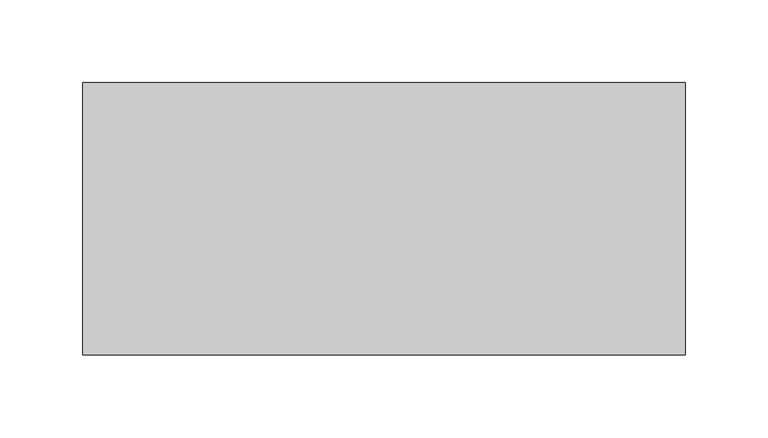
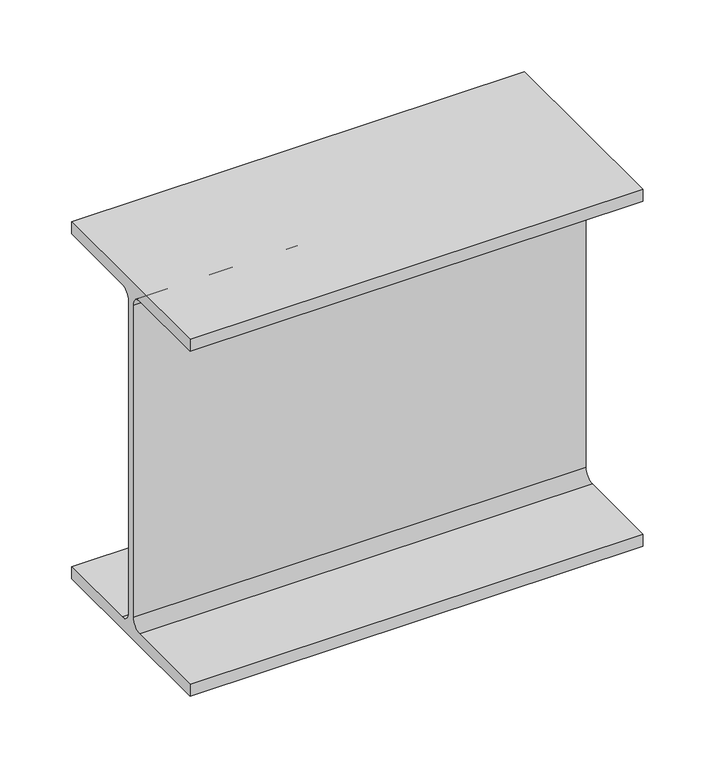
"""IFC4 building model written with IfcOpenShell, lengths in millimetres: beam geometry, Steel Beam_H-KSD3502 : H_SB_ASB_H-300x150x6.5x9."""

from ifc_helpers import new_model, si_unit, point, frame, frame_2d, origin, place, context, project, spatial, polyline, circle_curve, trimmed, segment, composite_curve, outline, extrude, source, transform, mapped, element, save


def beam_067efcca(model_context):
    return source(origin(), model_context, "Body", "SweptSolid", [
        extrude(outline(composite_curve([segment(polyline([(82.5, -141.5), (82.5, -151.7), (-82.5, -151.7), (-82.5, -141.5), (-11.9, -141.5)]), True, "CONTINUOUS"), segment(trimmed(circle_curve(frame_2d((-11.9, -132.6)), 8.9), [point((-11.9, -141.5))], [point((-3.0, -132.6))], True, "CARTESIAN"), True, "CONTINUOUS"), segment(polyline([(-3.0, -132.6), (-3.0, 132.6)]), True, "CONTINUOUS"), segment(trimmed(circle_curve(frame_2d((-11.9, 132.6)), 8.9), [point((-3.0, 132.6))], [point((-11.9, 141.5))], True, "CARTESIAN"), True, "CONTINUOUS"), segment(polyline([(-11.9, 141.5), (-82.5, 141.5), (-82.5, 151.7), (82.5, 151.7), (82.5, 141.5), (11.9, 141.5)]), True, "CONTINUOUS"), segment(trimmed(circle_curve(frame_2d((11.9, 132.6)), 8.9), [point((11.9, 141.5))], [point((3.0, 132.6))], True, "CARTESIAN"), True, "CONTINUOUS"), segment(polyline([(3.0, 132.6), (3.0, -132.6)]), True, "CONTINUOUS"), segment(trimmed(circle_curve(frame_2d((11.9, -132.6)), 8.9), [point((3.0, -132.6))], [point((11.9, -141.5))], True, "CARTESIAN"), True, "CONTINUOUS"), segment(polyline([(11.9, -141.5), (82.5, -141.5)]), True, "CONTINUOUS")], self_intersect=False)), frame((-282.3, 0.0, 0.0), z_axis=(1.0, 0.0, 0.0), x_axis=(0.0, 1.0, 0.0)), (0.0, 0.0, 1.0), 364.6),
    ])


if __name__ == "__main__":
    model = new_model("IFC4")
    model_context = context("Model", 3, world=origin())
    ifc_project = project(units=[si_unit("LENGTHUNIT", "METRE", prefix="MILLI")], contexts=[model_context])
    site = spatial("IfcSite", under=ifc_project)
    building = spatial("IfcBuilding", under=site)
    placement = place(None, origin())
    beam_shape = beam_067efcca(model_context)
    element("IfcBeam", 1, ObjectType="Steel Beam_H-KSD3502 : H_SB_ASB_H-300x150x6.5x9", at=placement, inside=building, context=model_context, shape_type="MappedRepresentation", body=[
        mapped(beam_shape, transform((0.0, 0.0, 0.0), x_axis=(1.0, 0.0, 0.0), y_axis=(0.0, 1.0, 0.0), z_axis=(0.0, 0.0, 1.0))),
    ])
    save(model, "model.ifc")

# Revit data of these elements
# Project information
#   Building Name = "STEAM TURBINE BUILDING"
#   H_Building Tag = "STB"
#   Project Status = "종결"
#   Client Name = "Therma Viayas Inc.\nTherma Viayas Inc.\nTherma Viayas Inc.\nTherma Viayas Inc."
#   Project Name = "Therma Visayas 2*150MW CFB Power Plant"
#   Project Number = "BEPH1402"
# Type "Steel Beam_H-KSD3502 : H_SB_ASB_H-300x150x6.5x9"
#   Width = 15.0 cm
#   Web Thickness = 0.65 cm
#   Web Fillet = 1.3 cm
#   Warping Constant = 107174.0 cm⁶
#   Torsional Moment of Inertia = 9.9539 cm⁴
#   Torsional Modulus = 1.0 cm³
#   Section Area = 46.78 cm²
#   Plastic Modulus weak axis = 105.0 cm³
#   Plastic Modulus strong axis = 542.0 cm³
#   Perimeter = 1.17 m²/m
#   Nominal Weight = 36.70 kgf/m
#   Moment of Inertia weak axis = 508.00 cm⁴
#   Moment of Inertia strong axis = 7210.00 cm⁴
#   Height = 30.0 cm
#   Flange Thickness = 0.9 cm
#   Elastic Modulus weak axis = 67.7 cm³
#   Elastic Modulus strong axis = 481.0 cm³
#   Centroid Vertical = 15.0 cm
#   Centroid Horizontal = 7.5 cm
#   Length [instance default] = 1.5240 m
#   Structural Material [instance default] = Steel, 45-345
#   Assembly Code = ""
# Element 1 (IfcBeam, "Steel Beam_H-KSD3502 : H_SB_ASB_H-300x150x6.5x9")
#   Structural Material = none
# Materials
#   "Steel, 45-345": class "Metal", colour RGB 189 187 185, transparency 0, Description = "Steel 345 MPa", Cost = 0
